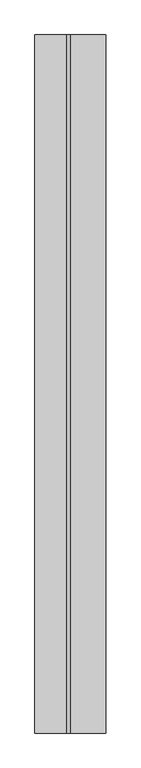
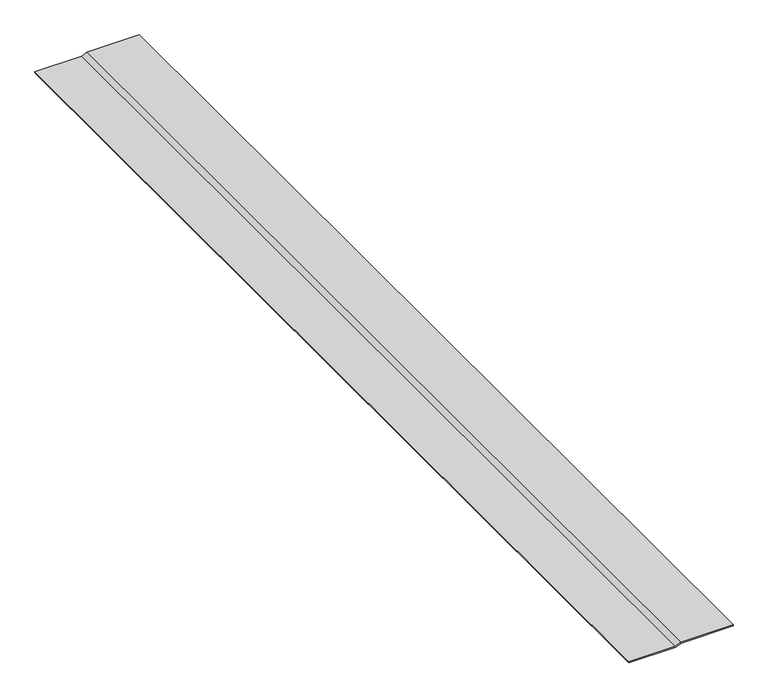
"""IFC4 building model written with IfcOpenShell, lengths in millimetres: proxy geometry, INTERPLY002 3772 : INTERPLY002 3772."""

import ifcopenshell
import ifcopenshell.guid

model = None  # the IFC model being written
_history = None  # IfcOwnerHistory: only IFC2X3 demands one
_inside = {}  # id of a spatial element -> (the spatial element, [elements in it])
_under = {}  # id of a project, library or spatial element -> (it, [spatial elements below it])
_declared = {}  # id of a project -> (the project, [libraries it declares])
_typed = {}  # id of a type object -> (the type object, [elements of that type])
_made_of = {}  # id of a material, layer set ... -> (it, [elements and type objects made of it])


def new_model(schema):
    """Start an empty IFC model of exactly this schema.

    Asked for "IFC4X3", IfcOpenShell would pick the latest addendum, in which some entities
    have other attributes; the version numbers below select the first issue.
    IFC2X3 requires an IfcOwnerHistory on every rooted entity: one is made here for all.
    """
    global model, _history
    if schema == "IFC4X3":
        model = ifcopenshell.file(schema_version=(4, 3, 0, 0))
    else:
        model = ifcopenshell.file(schema=schema)
    _inside.clear()
    _under.clear()
    _declared.clear()
    _typed.clear()
    _made_of.clear()
    _history = None
    if model.schema == "IFC2X3":
        org = make("IfcOrganization", Name="unknown")
        user = make(
            "IfcPersonAndOrganization",
            ThePerson=make("IfcPerson", FamilyName="unknown"),
            TheOrganization=org,
        )
        app = make(
            "IfcApplication",
            ApplicationDeveloper=org,
            Version="unknown",
            ApplicationFullName="unknown",
            ApplicationIdentifier="unknown",
        )
        _history = make(
            "IfcOwnerHistory",
            OwningUser=user,
            OwningApplication=app,
            ChangeAction="ADDED",
            CreationDate=0,
        )
    return model


def make(cls, **values):
    """One entity of the class cls with the attributes given. An attribute that is None is left unset."""
    return model.create_entity(
        cls, **{name: value for name, value in values.items() if value is not None}
    )


def rooted(cls, **values):
    """An entity with a GlobalId (a new one), such as an element, a storey or a relation."""
    return make(cls, GlobalId=ifcopenshell.guid.new(), OwnerHistory=_history, **values)


def si_unit(unit_type, name, prefix=None):
    """IfcSIUnit, for example si_unit("LENGTHUNIT", "METRE", prefix="MILLI")."""
    return make("IfcSIUnit", UnitType=unit_type, Prefix=prefix, Name=name)


def assignment(units):
    """IfcUnitAssignment: the units of a project."""
    return None if units is None else make("IfcUnitAssignment", Units=units)


def point(xyz):
    """IfcCartesianPoint."""
    return None if xyz is None else make("IfcCartesianPoint", Coordinates=xyz)


def direction(xyz):
    """IfcDirection."""
    return None if xyz is None else make("IfcDirection", DirectionRatios=xyz)


def frame(location, z_axis=None, x_axis=None):
    """IfcAxis2Placement3D, a coordinate frame: its origin and axes. An axis left out is left unset."""
    return make(
        "IfcAxis2Placement3D",
        Location=point(location),
        Axis=direction(z_axis),
        RefDirection=direction(x_axis),
    )


def origin():
    """The frame at (0, 0, 0) with its axes left unset."""
    return frame((0.0, 0.0, 0.0))


def place(relative_to, where):
    """IfcLocalPlacement: puts the frame where relative to a parent placement (None: the world)."""
    return make(
        "IfcLocalPlacement", PlacementRelTo=relative_to, RelativePlacement=where
    )


def context(
    kind, dimensions, precision=None, world=None, true_north=None, identifier=None
):
    """IfcGeometricRepresentationContext, for example the 3D "Model" context."""
    return make(
        "IfcGeometricRepresentationContext",
        ContextIdentifier=identifier,
        ContextType=kind,
        CoordinateSpaceDimension=dimensions,
        Precision=precision,
        WorldCoordinateSystem=world,
        TrueNorth=true_north,
    )


def project(units=None, contexts=None):
    """IfcProject with its units and contexts."""
    return rooted(
        "IfcProject",
        Name="project",
        RepresentationContexts=contexts,
        UnitsInContext=assignment(units),
    )


def spatial(cls, under=None, at=None, **own):
    """A site, building, storey or space (cls), placed at a placement, below another one or the project."""
    s = rooted(cls, ObjectPlacement=at, **own)
    if under is not None:
        _under.setdefault(under.id(), (under, []))[1].append(s)
    return s


def polyline(points):
    """IfcPolyline through the points."""
    return make("IfcPolyline", Points=[point(p) for p in points])


def outline(outer, holes=None, kind="AREA"):
    """IfcArbitraryClosedProfileDef: a profile drawn as a closed curve; with holes, ...WithVoids."""
    if holes is None:
        return make("IfcArbitraryClosedProfileDef", ProfileType=kind, OuterCurve=outer)
    return make(
        "IfcArbitraryProfileDefWithVoids",
        ProfileType=kind,
        OuterCurve=outer,
        InnerCurves=holes,
    )


def extrude(swept, where, along, depth):
    """IfcExtrudedAreaSolid: the profile swept, set in the frame where, extruded along a direction by depth."""
    return make(
        "IfcExtrudedAreaSolid",
        SweptArea=swept,
        Position=where,
        ExtrudedDirection=direction(along),
        Depth=depth,
    )


def shape(context_of_items, identifier, shape_type, items):
    """IfcShapeRepresentation: the items that make up one representation, for example the "Body"."""
    return make(
        "IfcShapeRepresentation",
        ContextOfItems=context_of_items,
        RepresentationIdentifier=identifier,
        RepresentationType=shape_type,
        Items=items,
    )


def source(mapping_origin, context_of_items, identifier, shape_type, items):
    """IfcRepresentationMap: a shape defined once, which mapped items show again and again."""
    return make(
        "IfcRepresentationMap",
        MappingOrigin=mapping_origin,
        MappedRepresentation=shape(context_of_items, identifier, shape_type, items),
    )


def transform(
    local_origin,
    x_axis=None,
    y_axis=None,
    z_axis=None,
    scale=None,
    scale2=None,
    scale3=None,
    uniform=True,
):
    """IfcCartesianTransformationOperator3D, or its non-uniform kind. x_axis, y_axis, z_axis: its Axis1, 2, 3."""
    if uniform:
        return make(
            "IfcCartesianTransformationOperator3D",
            Axis1=direction(x_axis),
            Axis2=direction(y_axis),
            LocalOrigin=point(local_origin),
            Scale=scale,
            Axis3=direction(z_axis),
        )
    return make(
        "IfcCartesianTransformationOperator3DnonUniform",
        Axis1=direction(x_axis),
        Axis2=direction(y_axis),
        LocalOrigin=point(local_origin),
        Scale=scale,
        Axis3=direction(z_axis),
        Scale2=scale2,
        Scale3=scale3,
    )


def mapped(mapping_source, mapping_target):
    """IfcMappedItem: shows the shape of a source again, moved by a transform."""
    return make(
        "IfcMappedItem", MappingSource=mapping_source, MappingTarget=mapping_target
    )


def made_of(thing, what):
    """Note that an element or type object is made of a material, layer set ...; save() writes the relation."""
    if what is not None:
        _made_of.setdefault(what.id(), (what, []))[1].append(thing)
    return thing


def element(
    cls,
    number,
    at=None,
    inside=None,
    cuts=None,
    type_object=None,
    material=None,
    context=None,
    identifier="Body",
    shape_type=None,
    held_by="IfcProductDefinitionShape",
    body=None,
    shapes=None,
    **own,
):
    """One element of the class cls, such as IfcWall. Its Tag is "e" and its number.

    at: its placement. inside: the storey or other place that contains it. cuts: it is an
    opening in that element (IfcRelVoidsElement). A single representation is given by context,
    identifier, shape_type and body (its items); several are given by shapes. held_by: the class
    of the entity that holds the representations. save() writes the other relations.
    """
    e = rooted(cls, Tag="e%d" % number, ObjectPlacement=at, **own)
    if body is not None:
        shapes = [shape(context, identifier, shape_type, body)]
    if shapes is not None:
        e.Representation = make(held_by, Representations=shapes)
    if inside is not None:
        _inside.setdefault(inside.id(), (inside, []))[1].append(e)
    if cuts is not None:
        rooted(
            "IfcRelVoidsElement", RelatingBuildingElement=cuts, RelatedOpeningElement=e
        )
    if type_object is not None:
        _typed.setdefault(type_object.id(), (type_object, []))[1].append(e)
    return made_of(e, material)


def aggregate(whole, parts):
    """IfcRelAggregates: a whole, such as a stair, and the parts it consists of."""
    return rooted("IfcRelAggregates", RelatingObject=whole, RelatedObjects=parts)


def save(model, path):
    """Write the relations noted so far, then the file.

    IfcRelAggregates (storeys below a building ...), IfcRelContainedInSpatialStructure (elements
    in a storey), IfcRelDefinesByType, IfcRelAssociatesMaterial and IfcRelDeclares: one each for
    every whole, place, type object, material and project.
    """
    for whole, parts in _under.values():
        aggregate(whole, parts)
    for where, things in _inside.values():
        rooted(
            "IfcRelContainedInSpatialStructure",
            RelatedElements=things,
            RelatingStructure=where,
        )
    for kind, things in _typed.values():
        rooted("IfcRelDefinesByType", RelatedObjects=things, RelatingType=kind)
    for what, things in _made_of.values():
        rooted("IfcRelAssociatesMaterial", RelatedObjects=things, RelatingMaterial=what)
    for by, libraries in _declared.values():
        rooted("IfcRelDeclares", RelatingContext=by, RelatedDefinitions=libraries)
    model.write(path)


def generic_models_8be46f14(model_context):
    return source(origin(), model_context, "Body", "SweptSolid", [
        extrude(outline(polyline([(40265.8733085, -4491.2259186), (40261.1620854, -4501.7914992), (40261.1620854, -4592.5295682), (40258.8529944, -4592.5295682), (40258.8529944, -4501.3000079), (40263.5642176, -4490.7344272), (40263.5642176, -4389.4895292), (40265.8733085, -4389.4895292), (40265.8733085, -4491.2259186)])), frame((0.0, -1065.5906573, 0.0), z_axis=(0.0, 1.0, 0.0), x_axis=(0.0, 0.0, 1.0)), (0.0, 0.0, 1.0), 2000.25),
    ])


if __name__ == "__main__":
    model = new_model("IFC4")
    model_context = context("Model", 3, world=origin())
    ifc_project = project(units=[si_unit("LENGTHUNIT", "METRE", prefix="MILLI")], contexts=[model_context])
    site = spatial("IfcSite", under=ifc_project)
    building = spatial("IfcBuilding", under=site)
    placement = place(None, origin())
    generic_models_shape = generic_models_8be46f14(model_context)
    element("IfcBuildingElementProxy", 1, Name="INTERPLY002 3772 : INTERPLY002 3772", ObjectType="INTERPLY002 3772 : INTERPLY002 3772", at=placement, inside=building, context=model_context, shape_type="MappedRepresentation", body=[
        mapped(generic_models_shape, transform((0.0, 0.0, 0.0), x_axis=(1.0, 0.0, 0.0), y_axis=(0.0, 1.0, 0.0), z_axis=(0.0, 0.0, 1.0))),
    ])
    save(model, "model.ifc")

# Revit data of these elements
# Type "INTERPLY002 3772 : INTERPLY002 3772"
#   NameOverride = "INTERPLY002"
# Element 1 (IfcBuildingElementProxy, "INTERPLY002 3772 : INTERPLY002 3772")
#   Materials on its faces: "INTERPLY"
# Materials
#   "INTERPLY": class "Unassigned", colour RGB 115 115 172, transparency 0
